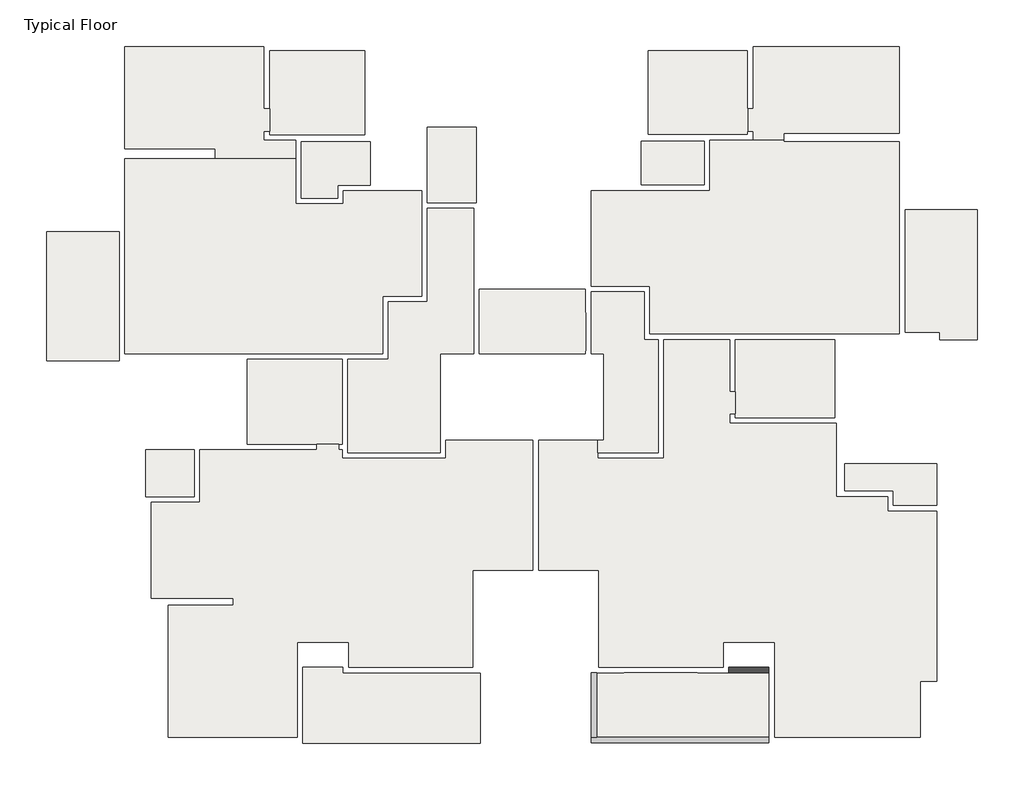
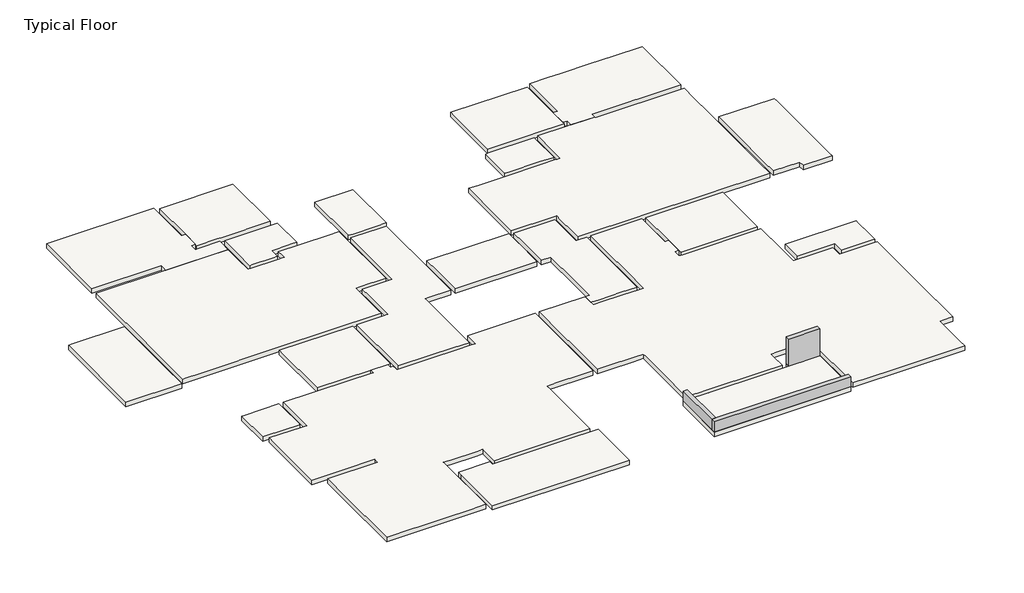
# One storey: 22 slabs, 3 beams.
"""IFC4 building model written with IfcOpenShell, lengths in millimetres."""

from ifc_helpers import new_model, si_unit, frame, origin, place, context, project, spatial, polyline, outline, extrude, faceted_brep, element, save

model = new_model("IFC4")

# Units and contexts
model_context = context("Model", 3, world=origin())
ifc_project = project(units=[si_unit("LENGTHUNIT", "METRE", prefix="MILLI")], contexts=[model_context])

# Site, building, storey
site = spatial("IfcSite", under=ifc_project)
building = spatial("IfcBuilding", under=site)
storey = spatial("IfcBuildingStorey", under=building, Name="Typical Floor", Elevation=3000.0)

# Beams
placement = place(None, origin())
element("IfcBeam", 1, ObjectType="Concrete Rectengular Beam : 20/133", at=placement, inside=storey, context=model_context, shape_type="Brep", body=[
    faceted_brep([(12927.905294, -11177.9835498, 4330.0), (12927.905294, -11177.9835498, 3000.0), (12927.905294, -11172.9835498, 3000.0), (12927.905294, -10977.9835498, 3000.0), (12927.905294, -10977.9835498, 4330.0), (11487.905294, -11177.9835498, 4330.0), (11487.905294, -10977.9835498, 4330.0), (11487.905294, -10977.9835498, 3000.0), (11487.905294, -11177.9835498, 3000.0)], [[[0, 1, 2, 3, 4]], [[5, 6, 7, 8]], [[4, 6, 5, 0]], [[3, 7, 6, 4]], [[1, 8, 7, 3, 2]], [[0, 5, 8, 1]]]),
])
element("IfcBeam", 2, ObjectType="Concrete Rectengular Beam : 20/50", at=placement, inside=storey, context=model_context, shape_type="Brep", body=[
    faceted_brep([(12927.905294, -13477.9835498, 3000.0), (12927.905294, -13477.9835498, 3500.0), (12927.905294, -13677.9835498, 3500.0), (12927.905294, -13677.9835498, 3000.0), (6765.405294, -13477.9835498, 3500.0), (6565.405294, -13477.9835498, 3500.0), (6565.405294, -13677.9835498, 3500.0), (6565.405294, -13677.9835498, 3000.0), (6565.405294, -13477.9835498, 3000.0), (6765.405294, -13477.9835498, 3000.0)], [[[0, 1, 2, 3]], [[2, 1, 4, 5, 6]], [[3, 2, 6, 7]], [[0, 3, 7, 8, 9]], [[1, 0, 9, 8, 5, 4]], [[6, 5, 8, 7]]]),
])
element("IfcBeam", 3, ObjectType="Concrete Rectengular Beam : 20/50", at=placement, inside=storey, context=model_context, shape_type="SweptSolid", body=[
    extrude(outline(polyline([(6565.405294, -11177.9835498), (6765.405294, -11177.9835498), (6765.405294, -13477.9835498), (6565.405294, -13477.9835498), (6565.405294, -11177.9835498)])), frame((0.0, 0.0, 3000.0), z_axis=(0.0, 0.0, 1.0), x_axis=(1.0, 0.0, 0.0)), (0.0, 0.0, 1.0), 500.0),
])

# Slabs
element("IfcSlab", 4, ObjectType="22", at=placement, inside=storey, context=model_context, shape_type="Brep", body=[
    faceted_brep([(2605.405294, -11177.9835498, 2780.0), (2605.405294, -13682.9835498, 2780.0), (-3754.594706, -13682.9835498, 2780.0), (-3754.594706, -11177.9835498, 2780.0), (-3754.594706, -10977.9835498, 2780.0), (-2314.594706, -10977.9835498, 2780.0), (-2314.594706, -11177.9835498, 2780.0), (-2114.594706, -11177.9835498, 2780.0), (-1184.594706, -11177.9835498, 2780.0), (1415.405294, -11177.9835498, 2780.0), (2605.405294, -13682.9835498, 3000.0), (2605.405294, -13482.9835498, 3000.0), (2605.405294, -11177.9835498, 3000.0), (2405.405294, -11177.9835498, 3000.0), (1415.405294, -11177.9835498, 3000.0), (-1184.594706, -11177.9835498, 3000.0), (-2114.594706, -11177.9835498, 3000.0), (-2314.594706, -11177.9835498, 3000.0), (-2314.594706, -10977.9835498, 3000.0), (-3754.594706, -10977.9835498, 3000.0), (-3754.594706, -11177.9835498, 3000.0), (-3754.594706, -13482.9835498, 3000.0), (-3754.594706, -13682.9835498, 3000.0)], [[[0, 1, 2, 3, 4, 5, 6, 7, 8, 9]], [[10, 11, 12, 13, 14, 15, 16, 17, 18, 19, 20, 21, 22]], [[1, 0, 12, 11, 10]], [[2, 1, 10, 22]], [[3, 2, 22, 21, 20]], [[4, 3, 20, 19]], [[5, 4, 19, 18]], [[6, 5, 18, 17]], [[6, 17, 16, 15, 14, 13, 12, 0, 9, 8, 7]]]),
])
element("IfcSlab", 5, ObjectType="22", at=placement, inside=storey, context=model_context, shape_type="Brep", body=[
    faceted_brep([(12927.905294, -13677.9835498, 2780.0), (6565.405294, -13677.9835498, 2780.0), (6565.405294, -11177.9835498, 2780.0), (7755.405294, -11177.9835498, 2780.0), (7755.405294, -11172.9835498, 2780.0), (10357.905294, -11172.9835498, 2780.0), (10357.905294, -11177.9835498, 2780.0), (11487.905294, -11177.9835498, 2780.0), (11487.905294, -10972.9835498, 2780.0), (12927.905294, -10972.9835498, 2780.0), (12927.905294, -11172.9835498, 2780.0), (6565.405294, -13677.9835498, 3000.0), (12927.905294, -13677.9835498, 3000.0), (12927.905294, -13477.9835498, 3000.0), (12927.905294, -11177.9835498, 3000.0), (12927.905294, -11172.9835498, 3000.0), (12927.905294, -10977.9835498, 3000.0), (12927.905294, -10972.9835498, 3000.0), (11487.905294, -10972.9835498, 3000.0), (11487.905294, -10977.9835498, 3000.0), (11487.905294, -11177.9835498, 3000.0), (10357.905294, -11177.9835498, 3000.0), (10357.905294, -11172.9835498, 3000.0), (7755.405294, -11172.9835498, 3000.0), (7755.405294, -11177.9835498, 3000.0), (6835.405294, -11177.9835498, 3000.0), (6765.405294, -11177.9835498, 3000.0), (6565.405294, -11177.9835498, 3000.0), (6565.405294, -13477.9835498, 3000.0)], [[[0, 1, 2, 3, 4, 5, 6, 7, 8, 9, 10]], [[11, 12, 13, 14, 15, 16, 17, 18, 19, 20, 21, 22, 23, 24, 25, 26, 27, 28]], [[1, 11, 28, 27, 2]], [[1, 0, 12, 11]], [[0, 10, 15, 14, 13, 12]], [[10, 9, 17, 16, 15]], [[17, 9, 8, 18]], [[4, 23, 22, 5]], [[2, 27, 26, 25, 24, 3]], [[3, 24, 23, 4]], [[6, 21, 20, 7]], [[21, 6, 5, 22]], [[7, 20, 19, 18, 8]]]),
])
element("IfcSlab", 6, ObjectType="22", at=placement, inside=storey, context=model_context, shape_type="Brep", body=[
    faceted_brep([(-4939.8370837, 11086.5624033, 2780.0), (-1534.8370837, 11086.5624033, 2780.0), (-1534.8370837, 8086.5624033, 2780.0), (-4939.8370837, 8086.5624033, 2780.0), (-4939.8370837, 8206.5624033, 2780.0), (-4939.8370837, 9006.5624033, 2780.0), (-1534.8370837, 11086.5624033, 3000.0), (-4939.8370837, 11086.5624033, 3000.0), (-4939.8370837, 9006.5624033, 3000.0), (-4939.8370837, 8206.5624033, 3000.0), (-4939.8370837, 8086.5624033, 3000.0), (-3999.8370837, 8086.5624033, 3000.0), (-3799.8370837, 8086.5624033, 3000.0), (-1534.8370837, 8086.5624033, 3000.0)], [[[0, 1, 2, 3, 4, 5]], [[6, 7, 8, 9, 10, 11, 12, 13]], [[1, 0, 7, 6]], [[1, 6, 13, 2]], [[7, 0, 5, 4, 3, 10, 9, 8]], [[10, 3, 2, 13, 12, 11]]]),
])
element("IfcSlab", 7, ObjectType="22", at=placement, inside=storey, context=model_context, shape_type="Brep", body=[
    faceted_brep([(-10119.6462524, 7575.1187953, 2780.0), (-10119.6462524, 11236.5624033, 2780.0), (-5139.8370837, 11236.5624033, 2780.0), (-5139.8370837, 9006.5624033, 2780.0), (-4939.8370837, 9006.5624033, 2780.0), (-4939.8370837, 8206.5624033, 2780.0), (-5139.8370837, 8206.5624033, 2780.0), (-5139.8370837, 7886.5624033, 2780.0), (-4939.8370837, 7886.5624033, 2780.0), (-3999.8370837, 7886.5624033, 2780.0), (-3999.8370837, 7215.1187953, 2780.0), (-6891.2699366, 7215.1187953, 2780.0), (-6891.2699366, 7575.1187953, 2780.0), (-10119.6462524, 11236.5624033, 3000.0), (-10119.6462524, 10130.5632806, 3000.0), (-10119.6462524, 8930.3987709, 3000.0), (-10119.6462524, 7575.1187953, 3000.0), (-6891.2699366, 7575.1187953, 3000.0), (-6891.2699366, 7215.1187953, 3000.0), (-3999.8370837, 7215.1187953, 3000.0), (-3999.8370837, 7726.5624033, 3000.0), (-3999.8370837, 7886.5624033, 3000.0), (-4939.8370837, 7886.5624033, 3000.0), (-5139.8370837, 7886.5624033, 3000.0), (-5139.8370837, 8206.5624033, 3000.0), (-4939.8370837, 8206.5624033, 3000.0), (-4939.8370837, 9006.5624033, 3000.0), (-5139.8370837, 9006.5624033, 3000.0), (-5139.8370837, 11236.5624033, 3000.0)], [[[0, 1, 2, 3, 4, 5, 6, 7, 8, 9, 10, 11, 12]], [[13, 14, 15, 16, 17, 18, 19, 20, 21, 22, 23, 24, 25, 26, 27, 28]], [[1, 0, 16, 15, 14, 13]], [[2, 1, 13, 28]], [[3, 2, 28, 27]], [[4, 3, 27, 26]], [[5, 4, 26, 25]], [[6, 5, 25, 24]], [[7, 6, 24, 23]], [[7, 23, 22, 21, 9, 8]], [[10, 9, 21, 20, 19]], [[11, 10, 19, 18]], [[12, 11, 18, 17]], [[0, 12, 17, 16]]]),
])
element("IfcSlab", 8, ObjectType="22", at=placement, inside=storey, context=model_context, shape_type="Brep", body=[
    faceted_brep([(508.320407, 6080.1520062, 2780.0), (508.320407, 2305.1520062, 2780.0), (-690.8131749, 2305.1520062, 2780.0), (-890.8131749, 2305.1520062, 2780.0), (-890.8131749, 1555.8429472, 2780.0), (-890.8131749, 556.7642019, 2780.0), (-890.8131749, 251.1884177, 2780.0), (-10119.6462524, 251.1884177, 2780.0), (-10119.6462524, 7215.1187953, 2780.0), (-6891.2699366, 7215.1187953, 2780.0), (-3999.8370837, 7215.1187953, 2780.0), (-3999.8370837, 6335.1520062, 2780.0), (-3999.8370837, 5815.1520062, 2780.0), (-3999.8370837, 5615.1520062, 2780.0), (-3696.679593, 5615.1520062, 2780.0), (-2696.679593, 5615.1520062, 2780.0), (-2301.679593, 5615.1520062, 2780.0), (-2301.679593, 5815.1520062, 2780.0), (-2301.679593, 6080.1520062, 2780.0), (-1171.679593, 6080.1520062, 2780.0), (28.320407, 6080.1520062, 2780.0), (508.320407, 2305.1520062, 3000.0), (508.320407, 6080.1520062, 3000.0), (28.320407, 6080.1520062, 3000.0), (-1171.679593, 6080.1520062, 3000.0), (-2301.679593, 6080.1520062, 3000.0), (-2301.679593, 5815.1520062, 3000.0), (-2301.679593, 5615.1520062, 3000.0), (-2696.679593, 5615.1520062, 3000.0), (-3696.679593, 5615.1520062, 3000.0), (-3999.8370837, 5615.1520062, 3000.0), (-3999.8370837, 5815.1520062, 3000.0), (-3999.8370837, 6335.1520062, 3000.0), (-3999.8370837, 7215.1187953, 3000.0), (-6891.2699366, 7215.1187953, 3000.0), (-10119.6462524, 7215.1187953, 3000.0), (-10119.6462524, 7055.0094311, 3000.0), (-10119.6462524, 5854.8449214, 3000.0), (-10119.6462524, 3780.4865094, 3000.0), (-10119.6462524, 1181.1884177, 3000.0), (-10119.6462524, 251.1884177, 3000.0), (-9999.6462524, 251.1884177, 3000.0), (-9290.9338154, 251.1884177, 3000.0), (-5740.9338154, 251.1884177, 3000.0), (-890.8131749, 251.1884177, 3000.0), (-890.8131749, 556.7642019, 3000.0), (-890.8131749, 1555.8429472, 3000.0), (-890.8131749, 2305.1520062, 3000.0), (-690.8131749, 2305.1520062, 3000.0)], [[[0, 1, 2, 3, 4, 5, 6, 7, 8, 9, 10, 11, 12, 13, 14, 15, 16, 17, 18, 19, 20]], [[21, 22, 23, 24, 25, 26, 27, 28, 29, 30, 31, 32, 33, 34, 35, 36, 37, 38, 39, 40, 41, 42, 43, 44, 45, 46, 47, 48]], [[30, 13, 12, 11, 10, 33, 32, 31]], [[13, 30, 29, 28, 27, 16, 15, 14]], [[16, 27, 26, 25, 18, 17]], [[18, 25, 24, 23, 22, 0, 20, 19]], [[1, 0, 22, 21]], [[1, 21, 48, 47, 3, 2]], [[3, 47, 46, 45, 44, 6, 5, 4]], [[7, 6, 44, 43, 42, 41, 40]], [[8, 7, 40, 39, 38, 37, 36, 35]], [[10, 9, 8, 35, 34, 33]]]),
])
element("IfcSlab", 9, ObjectType="22", at=placement, inside=storey, context=model_context, shape_type="Brep", body=[
    faceted_brep([(-12919.6462524, 4616.1884177, 2780.0), (-10319.6462524, 4616.1884177, 2780.0), (-10319.6462524, -12.6260152, 2780.0), (-12919.6462524, -12.6260152, 2780.0), (-12919.6462524, 4616.1884177, 3000.0), (-12919.6462524, 187.3739848, 3000.0), (-12919.6462524, -12.6260152, 3000.0), (-10319.6462524, -12.6260152, 3000.0), (-10319.6462524, 187.3739848, 3000.0), (-10319.6462524, 251.1884177, 3000.0), (-10319.6462524, 1181.1884177, 3000.0), (-10319.6462524, 3780.4865094, 3000.0), (-10319.6462524, 4416.1884177, 3000.0), (-10319.6462524, 4616.1884177, 3000.0), (-12719.6462524, 4616.1884177, 3000.0)], [[[0, 1, 2, 3]], [[4, 5, 6, 7, 8, 9, 10, 11, 12, 13, 14]], [[1, 0, 4, 14, 13]], [[2, 1, 13, 12, 11, 10, 9, 8, 7]], [[3, 2, 7, 6]], [[0, 3, 6, 5, 4]]]),
])
element("IfcSlab", 10, ObjectType="22", at=placement, inside=storey, context=model_context, shape_type="Brep", body=[
    faceted_brep([(-1339.8370837, 7836.5624033, 2780.0), (-1339.8370837, 6280.1520062, 2780.0), (-2301.679593, 6280.1520062, 2780.0), (-2501.679593, 6280.1520062, 2780.0), (-2501.679593, 5815.1520062, 2780.0), (-3799.8370837, 5815.1520062, 2780.0), (-3799.8370837, 7836.5624033, 2780.0), (-1339.8370837, 6280.1520062, 3000.0), (-1339.8370837, 7836.068874, 3000.0), (-1339.8370837, 7836.5624033, 3000.0), (-3799.8370837, 7836.5624033, 3000.0), (-3799.8370837, 7726.5624033, 3000.0), (-3799.8370837, 6335.1520062, 3000.0), (-3799.8370837, 5815.1520062, 3000.0), (-3696.679593, 5815.1520062, 3000.0), (-2696.679593, 5815.1520062, 3000.0), (-2501.679593, 5815.1520062, 3000.0), (-2501.679593, 6280.1520062, 3000.0), (-2301.679593, 6280.1520062, 3000.0), (-1489.8370837, 6280.1520062, 3000.0)], [[[0, 1, 2, 3, 4, 5, 6]], [[7, 8, 9, 10, 11, 12, 13, 14, 15, 16, 17, 18, 19]], [[1, 0, 9, 8, 7]], [[1, 7, 19, 18, 17, 3, 2]], [[4, 3, 17, 16]], [[5, 4, 16, 15, 14, 13]], [[6, 5, 13, 12, 11, 10]], [[0, 6, 10, 9]]]),
])
element("IfcSlab", 11, ObjectType="22", at=placement, inside=storey, context=model_context, shape_type="Brep", body=[
    faceted_brep([(8357.905294, 7842.0164502, 2780.0), (10617.905294, 7842.0164502, 2780.0), (10617.905294, 6284.3445962, 2780.0), (8357.905294, 6284.3445962, 2780.0), (8357.905294, 7842.0164502, 3000.0), (8357.905294, 6284.3445962, 3000.0), (8507.905294, 6284.3445962, 3000.0), (9959.9948169, 6284.3445962, 3000.0), (10569.9948169, 6284.3445962, 3000.0), (10617.905294, 6284.3445962, 3000.0), (10617.905294, 6354.3445962, 3000.0), (10617.905294, 7752.0164502, 3000.0), (10617.905294, 7842.0164502, 3000.0), (8507.905294, 7842.0164502, 3000.0)], [[[0, 1, 2, 3]], [[4, 5, 6, 7, 8, 9, 10, 11, 12, 13]], [[1, 0, 4, 13, 12]], [[2, 1, 12, 11, 10, 9]], [[3, 2, 9, 8, 7, 6, 5]], [[0, 3, 5, 4]]]),
])
element("IfcSlab", 12, ObjectType="22", at=placement, inside=storey, context=model_context, shape_type="Brep", body=[
    faceted_brep([(8607.905294, 8092.0164502, 2780.0), (8607.905294, 11082.0164502, 2780.0), (12157.905294, 11082.0164502, 2780.0), (12157.905294, 9012.0164502, 2780.0), (12162.905294, 9012.0164502, 2780.0), (12162.905294, 8212.0164502, 2780.0), (12157.905294, 8212.0164502, 2780.0), (12157.905294, 8092.0164502, 2780.0), (8607.905294, 11082.0164502, 3000.0), (8607.905294, 8092.0164502, 3000.0), (10617.905294, 8092.0164502, 3000.0), (10817.905294, 8092.0164502, 3000.0), (12157.905294, 8092.0164502, 3000.0), (12157.905294, 8212.0164502, 3000.0), (12162.905294, 8212.0164502, 3000.0), (12162.905294, 9012.0164502, 3000.0), (12157.905294, 9012.0164502, 3000.0), (12157.905294, 11082.0164502, 3000.0)], [[[0, 1, 2, 3, 4, 5, 6, 7]], [[8, 9, 10, 11, 12, 13, 14, 15, 16, 17]], [[4, 15, 14, 5]], [[9, 0, 7, 12, 11, 10]], [[1, 0, 9, 8]], [[1, 8, 17, 2]], [[16, 3, 2, 17]], [[3, 16, 15, 4]], [[6, 13, 12, 7]], [[13, 6, 5, 14]]]),
])
element("IfcSlab", 13, ObjectType="22", at=placement, inside=storey, context=model_context, shape_type="Brep", body=[
    faceted_brep([(12357.905294, 9012.0164502, 2780.0), (12357.905294, 11232.0164502, 2780.0), (17597.905294, 11232.0164502, 2780.0), (17597.905294, 8132.0164502, 2780.0), (13457.905294, 8132.0164502, 2780.0), (13457.905294, 7892.0164502, 2780.0), (12357.905294, 7892.0164502, 2780.0), (12357.905294, 8212.0164502, 2780.0), (12162.905294, 8212.0164502, 2780.0), (12162.905294, 9012.0164502, 2780.0), (12357.905294, 11232.0164502, 3000.0), (12357.905294, 9012.0164502, 3000.0), (12162.905294, 9012.0164502, 3000.0), (12162.905294, 8212.0164502, 3000.0), (12357.905294, 8212.0164502, 3000.0), (12357.905294, 7892.0164502, 3000.0), (13457.905294, 7892.0164502, 3000.0), (13457.905294, 8132.0164502, 3000.0), (17597.905294, 8132.0164502, 3000.0), (17597.905294, 11232.0164502, 3000.0), (16317.905294, 11232.0164502, 3000.0), (15097.905294, 11232.0164502, 3000.0), (13857.905294, 11232.0164502, 3000.0), (13257.905294, 11232.0164502, 3000.0)], [[[0, 1, 2, 3, 4, 5, 6, 7, 8, 9]], [[10, 11, 12, 13, 14, 15, 16, 17, 18, 19, 20, 21, 22, 23]], [[7, 14, 13, 8]], [[11, 0, 9, 12]], [[1, 0, 11, 10]], [[2, 1, 10, 23, 22, 21, 20, 19]], [[3, 2, 19, 18]], [[4, 3, 18, 17]], [[5, 4, 17, 16]], [[6, 5, 16, 15]], [[7, 6, 15, 14]], [[9, 8, 13, 12]]]),
])
element("IfcSlab", 14, ObjectType="22", at=placement, inside=storey, context=model_context, shape_type="Brep", body=[
    faceted_brep([(10817.905294, 7892.0164502, 2780.0), (12357.905294, 7892.0164502, 2780.0), (13457.905294, 7892.0164502, 2780.0), (13457.905294, 7832.0164502, 2780.0), (17597.905294, 7832.0164502, 2780.0), (17597.905294, 1022.0164502, 2780.0), (17597.905294, 952.0164502, 2780.0), (8663.320407, 952.0164502, 2780.0), (8663.320407, 1352.0164502, 2780.0), (8663.320407, 2355.1520062, 2780.0), (8663.320407, 2655.1520062, 2780.0), (8463.320407, 2655.1520062, 2780.0), (6563.320407, 2655.1520062, 2780.0), (6563.320407, 6084.3445962, 2780.0), (7043.320407, 6084.3445962, 2780.0), (8239.9948169, 6084.3445962, 2780.0), (9959.9948169, 6084.3445962, 2780.0), (10569.9948169, 6084.3445962, 2780.0), (10617.905294, 6084.3445962, 2780.0), (10817.905294, 6084.3445962, 2780.0), (10817.905294, 6354.3445962, 2780.0), (10817.905294, 7752.0164502, 2780.0), (13457.905294, 7892.0164502, 3000.0), (12357.905294, 7892.0164502, 3000.0), (12157.905294, 7892.0164502, 3000.0), (10817.905294, 7892.0164502, 3000.0), (10817.905294, 7752.0164502, 3000.0), (10817.905294, 6354.3445962, 3000.0), (10817.905294, 6084.3445962, 3000.0), (10617.905294, 6084.3445962, 3000.0), (10569.9948169, 6084.3445962, 3000.0), (9959.9948169, 6084.3445962, 3000.0), (8239.9948169, 6084.3445962, 3000.0), (7043.320407, 6084.3445962, 3000.0), (6563.320407, 6084.3445962, 3000.0), (6563.320407, 2655.1520062, 3000.0), (8463.320407, 2655.1520062, 3000.0), (8663.320407, 2655.1520062, 3000.0), (8663.320407, 2355.1520062, 3000.0), (8663.320407, 1352.0164502, 3000.0), (8663.320407, 952.0164502, 3000.0), (17597.905294, 952.0164502, 3000.0), (17597.905294, 1022.0164502, 3000.0), (17597.905294, 1732.0164502, 3000.0), (17597.905294, 4332.0164502, 3000.0), (17597.905294, 5872.0164502, 3000.0), (17597.905294, 7092.0164502, 3000.0), (17597.905294, 7832.0164502, 3000.0), (13457.905294, 7832.0164502, 3000.0)], [[[0, 1, 2, 3, 4, 5, 6, 7, 8, 9, 10, 11, 12, 13, 14, 15, 16, 17, 18, 19, 20, 21]], [[22, 23, 24, 25, 26, 27, 28, 29, 30, 31, 32, 33, 34, 35, 36, 37, 38, 39, 40, 41, 42, 43, 44, 45, 46, 47, 48]], [[28, 19, 18, 17, 16, 15, 14, 13, 34, 33, 32, 31, 30, 29]], [[19, 28, 27, 26, 25, 0, 21, 20]], [[2, 1, 0, 25, 24, 23, 22]], [[3, 2, 22, 48]], [[4, 3, 48, 47]], [[5, 4, 47, 46, 45, 44, 43, 42]], [[6, 5, 42, 41]], [[7, 6, 41, 40]], [[7, 40, 39, 38, 37, 10, 9, 8]], [[10, 37, 36, 35, 12, 11]], [[13, 12, 35, 34]]]),
])
element("IfcSlab", 15, ObjectType="22", at=placement, inside=storey, context=model_context, shape_type="Brep", body=[
    faceted_brep([(17797.905294, 5405.0203984, 2780.0), (20388.2392489, 5405.0203984, 2780.0), (20388.2392489, 1022.0164502, 2780.0), (20388.2392489, 752.0164502, 2780.0), (19037.905294, 752.0164502, 2780.0), (19037.905294, 1022.0164502, 2780.0), (17797.905294, 1022.0164502, 2780.0), (20388.2392489, 5405.0203984, 3000.0), (17797.905294, 5405.0203984, 3000.0), (17797.905294, 5205.0203984, 3000.0), (17797.905294, 4332.0164502, 3000.0), (17797.905294, 1732.0164502, 3000.0), (17797.905294, 1022.0164502, 3000.0), (19037.905294, 1022.0164502, 3000.0), (19037.905294, 752.0164502, 3000.0), (20188.2392489, 752.0164502, 3000.0), (20388.2392489, 752.0164502, 3000.0), (20388.2392489, 1022.0164502, 3000.0), (20388.2392489, 5205.0203984, 3000.0)], [[[0, 1, 2, 3, 4, 5, 6]], [[7, 8, 9, 10, 11, 12, 13, 14, 15, 16, 17, 18]], [[1, 0, 8, 7]], [[2, 1, 7, 18, 17]], [[6, 5, 13, 12]], [[0, 6, 12, 11, 10, 9, 8]], [[3, 2, 17, 16]], [[4, 3, 16, 15, 14]], [[5, 4, 14, 13]]]),
])
element("IfcSlab", 16, ObjectType="22", at=placement, inside=storey, context=model_context, shape_type="Brep", body=[
    faceted_brep([(2460.820407, 8355.1520062, 2780.0), (2460.820407, 5655.8758492, 2780.0), (708.320407, 5655.8758492, 2780.0), (708.320407, 8355.1520062, 2780.0), (2460.820407, 8355.1520062, 3000.0), (708.320407, 8355.1520062, 3000.0), (708.320407, 5655.8758492, 3000.0), (909.4061714, 5655.8758492, 3000.0), (2013.320407, 5655.8758492, 3000.0), (2460.820407, 5655.8758492, 3000.0)], [[[0, 1, 2, 3]], [[4, 5, 6, 7, 8, 9]], [[1, 0, 4, 9]], [[2, 1, 9, 8, 7, 6]], [[3, 2, 6, 5]], [[0, 3, 5, 4]]]),
])
element("IfcSlab", 17, ObjectType="22", at=placement, inside=storey, context=model_context, shape_type="Brep", body=[
    faceted_brep([(1160.820407, 252.3535615, 2780.0), (1160.820407, -3294.0144776, 2780.0), (-2136.5139865, -3294.0144776, 2780.0), (-2136.5139865, 51.1884177, 2780.0), (-890.8131749, 51.1884177, 2780.0), (-690.8131749, 51.1884177, 2780.0), (-690.8131749, 556.7642019, 2780.0), (-690.8131749, 1555.8429472, 2780.0), (-690.8131749, 2105.1520062, 2780.0), (708.320407, 2105.1520062, 2780.0), (708.320407, 2305.1520062, 2780.0), (708.320407, 5455.8758492, 2780.0), (2360.820407, 5455.8758492, 2780.0), (2360.820407, 1705.8758492, 2780.0), (2363.3932055, 1705.8758492, 2780.0), (2363.3932055, 352.3535615, 2780.0), (2360.820407, 352.3535615, 2780.0), (2360.820407, 252.3535615, 2780.0), (1360.820407, 252.3535615, 2780.0), (1160.820407, -3294.0144776, 3000.0), (1160.820407, 252.3535615, 3000.0), (1360.820407, 252.3535615, 3000.0), (2360.820407, 252.3535615, 3000.0), (2360.820407, 352.3535615, 3000.0), (2363.3932055, 352.3535615, 3000.0), (2363.3932055, 1705.8758492, 3000.0), (2360.820407, 1705.8758492, 3000.0), (2360.820407, 5455.8758492, 3000.0), (2013.320407, 5455.8758492, 3000.0), (909.4061714, 5455.8758492, 3000.0), (708.320407, 5455.8758492, 3000.0), (708.320407, 2305.1520062, 3000.0), (708.320407, 2105.1520062, 3000.0), (-690.8131749, 2105.1520062, 3000.0), (-690.8131749, 1555.8429472, 3000.0), (-690.8131749, 556.7642019, 3000.0), (-690.8131749, 51.1884177, 3000.0), (-890.8131749, 51.1884177, 3000.0), (-2136.5139865, 51.1884177, 3000.0), (-2136.5139865, -3294.0144776, 3000.0), (-591.3286388, -3294.0144776, 3000.0), (410.820407, -3294.0144776, 3000.0)], [[[0, 1, 2, 3, 4, 5, 6, 7, 8, 9, 10, 11, 12, 13, 14, 15, 16, 17, 18]], [[19, 20, 21, 22, 23, 24, 25, 26, 27, 28, 29, 30, 31, 32, 33, 34, 35, 36, 37, 38, 39, 40, 41]], [[14, 25, 24, 15]], [[20, 0, 18, 17, 22, 21]], [[1, 0, 20, 19]], [[2, 1, 19, 41, 40, 39]], [[3, 2, 39, 38]], [[3, 38, 37, 36, 5, 4]], [[5, 36, 35, 34, 33, 8, 7, 6]], [[9, 8, 33, 32]], [[9, 32, 31, 30, 11, 10]], [[11, 30, 29, 28, 27, 12]], [[26, 13, 12, 27]], [[13, 26, 25, 14]], [[16, 23, 22, 17]], [[23, 16, 15, 24]]]),
])
element("IfcSlab", 18, ObjectType="22", at=placement, inside=storey, context=model_context, shape_type="Brep", body=[
    faceted_brep([(2560.820407, 252.3535615, 2780.0), (2560.820407, 2545.8758492, 2780.0), (6363.320407, 2545.8758492, 2780.0), (6363.320407, 1705.1520062, 2780.0), (6368.320407, 1705.1520062, 2780.0), (6368.320407, 352.3535615, 2780.0), (6363.320407, 352.3535615, 2780.0), (6363.320407, 252.3535615, 2780.0), (2560.820407, 2545.8758492, 3000.0), (2560.820407, 1705.8758492, 3000.0), (2560.820407, 352.3535615, 3000.0), (2560.820407, 252.3535615, 3000.0), (6363.320407, 252.3535615, 3000.0), (6363.320407, 352.3535615, 3000.0), (6368.320407, 352.3535615, 3000.0), (6368.320407, 1705.1520062, 3000.0), (6363.320407, 1705.1520062, 3000.0), (6363.320407, 2545.8758492, 3000.0)], [[[0, 1, 2, 3, 4, 5, 6, 7]], [[8, 9, 10, 11, 12, 13, 14, 15, 16, 17]], [[4, 15, 14, 5]], [[11, 0, 7, 12]], [[1, 0, 11, 10, 9, 8]], [[1, 8, 17, 2]], [[16, 3, 2, 17]], [[3, 16, 15, 4]], [[6, 13, 12, 7]], [[13, 6, 5, 14]]]),
])
element("IfcSlab", 19, ObjectType="22", at=placement, inside=storey, context=model_context, shape_type="Brep", body=[
    faceted_brep([(8963.320407, 752.0164502, 2780.0), (8963.320407, -3297.9835498, 2780.0), (6810.820407, -3297.9835498, 2780.0), (6810.820407, -2847.6464385, 2780.0), (7010.820407, -2847.6464385, 2780.0), (7010.820407, -2447.6464385, 2780.0), (7010.820407, -1347.6464385, 2780.0), (7010.820407, 52.3535615, 2780.0), (7010.820407, 252.3535615, 2780.0), (6563.320407, 252.3535615, 2780.0), (6563.320407, 2455.1520062, 2780.0), (8463.320407, 2455.1520062, 2780.0), (8463.320407, 2355.1520062, 2780.0), (8463.320407, 1352.0164502, 2780.0), (8463.320407, 752.0164502, 2780.0), (8663.320407, 752.0164502, 2780.0), (8963.320407, -3297.9835498, 3000.0), (8963.320407, 752.0164502, 3000.0), (8663.320407, 752.0164502, 3000.0), (8463.320407, 752.0164502, 3000.0), (8463.320407, 1352.0164502, 3000.0), (8463.320407, 2355.1520062, 3000.0), (8463.320407, 2455.1520062, 3000.0), (6563.320407, 2455.1520062, 3000.0), (6563.320407, 1705.1520062, 3000.0), (6563.320407, 352.3535615, 3000.0), (6563.320407, 252.3535615, 3000.0), (7010.820407, 252.3535615, 3000.0), (7010.820407, 52.3535615, 3000.0), (7010.820407, -1347.6464385, 3000.0), (7010.820407, -2447.6464385, 3000.0), (7010.820407, -2847.6464385, 3000.0), (6810.820407, -2847.6464385, 3000.0), (6810.820407, -3297.9835498, 3000.0), (7210.820407, -3297.9835498, 3000.0), (8213.320407, -3297.9835498, 3000.0)], [[[0, 1, 2, 3, 4, 5, 6, 7, 8, 9, 10, 11, 12, 13, 14, 15]], [[16, 17, 18, 19, 20, 21, 22, 23, 24, 25, 26, 27, 28, 29, 30, 31, 32, 33, 34, 35]], [[19, 14, 13, 12, 11, 22, 21, 20]], [[14, 19, 18, 17, 0, 15]], [[1, 0, 17, 16]], [[2, 1, 16, 35, 34, 33]], [[3, 2, 33, 32]], [[4, 3, 32, 31]], [[4, 31, 30, 29, 28, 27, 8, 7, 6, 5]], [[9, 8, 27, 26]], [[10, 9, 26, 25, 24, 23]], [[11, 10, 23, 22]]]),
])
element("IfcSlab", 20, ObjectType="22", at=placement, inside=storey, context=model_context, shape_type="Brep", body=[
    faceted_brep([(-7634.594706, -3194.7427075, 2780.0), (-7634.594706, -4872.9835498, 2780.0), (-9365.9338154, -4872.9835498, 2780.0), (-9365.9338154, -3194.7427075, 2780.0), (-7634.594706, -3194.7427075, 3000.0), (-9214.7328942, -3194.7427075, 3000.0), (-9364.7328942, -3194.7427075, 3000.0), (-9365.9338154, -3194.7427075, 3000.0), (-9365.9338154, -4872.9835498, 3000.0), (-9364.7328942, -4872.9835498, 3000.0), (-9214.7328942, -4872.9835498, 3000.0), (-7634.594706, -4872.9835498, 3000.0), (-7634.594706, -4812.9835498, 3000.0), (-7634.594706, -3392.9835498, 3000.0)], [[[0, 1, 2, 3]], [[4, 5, 6, 7, 8, 9, 10, 11, 12, 13]], [[1, 0, 4, 13, 12, 11]], [[2, 1, 11, 10, 9, 8]], [[3, 2, 8, 7]], [[0, 3, 7, 6, 5, 4]]]),
])
element("IfcSlab", 21, ObjectType="22", at=placement, inside=storey, context=model_context, shape_type="Brep", body=[
    faceted_brep([(-5740.9338154, -2994.7427075, 2780.0), (-5740.9338154, 51.1884177, 2780.0), (-2336.5139865, 51.1884177, 2780.0), (-2336.5139865, -2994.0144776, 2780.0), (-2456.1345173, -2994.0144776, 2780.0), (-2456.1345173, -2994.7427075, 2780.0), (-3252.010806, -2994.7427075, 2780.0), (-5740.9338154, 51.1884177, 3000.0), (-5740.9338154, -18.8115823, 3000.0), (-5740.9338154, -2994.7427075, 3000.0), (-3252.010806, -2994.7427075, 3000.0), (-2456.1345173, -2994.7427075, 3000.0), (-2456.1345173, -2994.0144776, 3000.0), (-2336.5139865, -2994.0144776, 3000.0), (-2336.5139865, 51.1884177, 3000.0)], [[[0, 1, 2, 3, 4, 5, 6]], [[7, 8, 9, 10, 11, 12, 13, 14]], [[2, 14, 13, 3]], [[9, 0, 6, 5, 11, 10]], [[1, 0, 9, 8, 7]], [[2, 1, 7, 14]], [[12, 4, 3, 13]], [[4, 12, 11, 5]]]),
])
element("IfcSlab", 22, ObjectType="22", at=placement, inside=storey, context=model_context, shape_type="Brep", body=[
    faceted_brep([(15289.9526685, 752.0164502, 2780.0), (15289.9526685, -2047.9835498, 2780.0), (11717.905294, -2047.9835498, 2780.0), (11717.905294, -1907.9835498, 2780.0), (11717.905294, -1107.9835498, 2780.0), (11717.905294, 752.0164502, 2780.0), (15289.9526685, 752.0164502, 3000.0), (11717.905294, 752.0164502, 3000.0), (11717.905294, -1107.9835498, 3000.0), (11717.905294, -1907.9835498, 3000.0), (11717.905294, -2047.9835498, 3000.0), (15289.9526685, -2047.9835498, 3000.0)], [[[0, 1, 2, 3, 4, 5]], [[6, 7, 8, 9, 10, 11]], [[1, 0, 6, 11]], [[2, 1, 11, 10]], [[5, 4, 3, 2, 10, 9, 8, 7]], [[0, 5, 7, 6]]]),
])
element("IfcSlab", 23, ObjectType="22", at=placement, inside=storey, context=model_context, shape_type="Brep", body=[
    faceted_brep([(18937.905294, -3693.5538503, 2780.0), (18937.905294, -4662.9835498, 2780.0), (18937.905294, -5182.9835498, 2780.0), (17377.905294, -5182.9835498, 2780.0), (17377.905294, -4862.9835498, 2780.0), (17377.905294, -4662.9835498, 2780.0), (16897.905294, -4662.9835498, 2780.0), (16277.905294, -4662.9835498, 2780.0), (15639.9526685, -4662.9835498, 2780.0), (15639.9526685, -3693.5538503, 2780.0), (18937.905294, -4662.9835498, 3000.0), (18937.905294, -3843.5538503, 3000.0), (18937.905294, -3693.5538503, 3000.0), (15639.9526685, -3693.5538503, 3000.0), (15639.9526685, -3843.5538503, 3000.0), (15639.9526685, -4662.9835498, 3000.0), (16277.905294, -4662.9835498, 3000.0), (16897.905294, -4662.9835498, 3000.0), (17377.905294, -4662.9835498, 3000.0), (17377.905294, -4862.9835498, 3000.0), (17377.905294, -5182.9835498, 3000.0), (17457.905294, -5182.9835498, 3000.0), (18857.905294, -5182.9835498, 3000.0), (18937.905294, -5182.9835498, 3000.0)], [[[0, 1, 2, 3, 4, 5, 6, 7, 8, 9]], [[10, 11, 12, 13, 14, 15, 16, 17, 18, 19, 20, 21, 22, 23]], [[1, 0, 12, 11, 10]], [[2, 1, 10, 23]], [[3, 2, 23, 22, 21, 20]], [[3, 20, 19, 18, 5, 4]], [[5, 18, 17, 16, 15, 8, 7, 6]], [[9, 8, 15, 14, 13]], [[0, 9, 13, 12]]]),
])
element("IfcSlab", 24, ObjectType="22", at=placement, inside=storey, context=model_context, shape_type="Brep", body=[
    faceted_brep([(11517.905294, -1107.9835498, 2780.0), (11717.905294, -1107.9835498, 2780.0), (11717.905294, -1907.9835498, 2780.0), (11517.905294, -1907.9835498, 2780.0), (11517.905294, -2247.9835498, 2780.0), (11717.905294, -2247.9835498, 2780.0), (15339.9526685, -2247.9835498, 2780.0), (15339.9526685, -2447.9835498, 2780.0), (15339.9526685, -3647.9835498, 2780.0), (15339.9526685, -4662.9835498, 2780.0), (15339.9526685, -4862.9835498, 2780.0), (16277.905294, -4862.9835498, 2780.0), (16897.905294, -4862.9835498, 2780.0), (17177.905294, -4862.9835498, 2780.0), (17177.905294, -5182.9835498, 2780.0), (17177.905294, -5382.9835498, 2780.0), (17457.905294, -5382.9835498, 2780.0), (18857.905294, -5382.9835498, 2780.0), (18937.905294, -5382.9835498, 2780.0), (18937.905294, -11472.9835498, 2780.0), (18537.905294, -11472.9835498, 2780.0), (18337.905294, -11472.9835498, 2780.0), (18337.905294, -12447.9835498, 2780.0), (18337.905294, -13047.9835498, 2780.0), (18337.905294, -13477.9835498, 2780.0), (13127.905294, -13477.9835498, 2780.0), (13127.905294, -10277.9835498, 2780.0), (13127.905294, -10077.9835498, 2780.0), (12807.905294, -10077.9835498, 2780.0), (11607.905294, -10077.9835498, 2780.0), (11287.905294, -10077.9835498, 2780.0), (11287.905294, -10277.9835498, 2780.0), (11287.905294, -10977.9835498, 2780.0), (10357.905294, -10977.9835498, 2780.0), (7755.405294, -10977.9835498, 2780.0), (6835.405294, -10977.9835498, 2780.0), (6835.405294, -7702.9835498, 2780.0), (6835.405294, -7502.9835498, 2780.0), (6385.405294, -7502.9835498, 2780.0), (5185.405294, -7502.9835498, 2780.0), (4685.405294, -7502.9835498, 2780.0), (4685.405294, -2847.6464385, 2780.0), (6810.820407, -2847.6464385, 2780.0), (6810.820407, -3297.9835498, 2780.0), (6810.820407, -3497.9835498, 2780.0), (7210.820407, -3497.9835498, 2780.0), (8213.320407, -3497.9835498, 2780.0), (8963.320407, -3497.9835498, 2780.0), (9163.320407, -3497.9835498, 2780.0), (9163.320407, 752.0164502, 2780.0), (11517.905294, 752.0164502, 2780.0), (11717.905294, -1107.9835498, 3000.0), (11517.905294, -1107.9835498, 3000.0), (11517.905294, 752.0164502, 3000.0), (9163.320407, 752.0164502, 3000.0), (9163.320407, -3497.9835498, 3000.0), (8963.320407, -3497.9835498, 3000.0), (8213.320407, -3497.9835498, 3000.0), (7210.820407, -3497.9835498, 3000.0), (6810.820407, -3497.9835498, 3000.0), (6810.820407, -3297.9835498, 3000.0), (6810.820407, -2847.6464385, 3000.0), (4685.405294, -2847.6464385, 3000.0), (4685.405294, -7502.9835498, 3000.0), (5185.405294, -7502.9835498, 3000.0), (6385.405294, -7502.9835498, 3000.0), (6835.405294, -7502.9835498, 3000.0), (6835.405294, -7702.9835498, 3000.0), (6835.405294, -10977.9835498, 3000.0), (7755.405294, -10977.9835498, 3000.0), (10357.905294, -10977.9835498, 3000.0), (11287.905294, -10977.9835498, 3000.0), (11287.905294, -10277.9835498, 3000.0), (11287.905294, -10077.9835498, 3000.0), (11607.905294, -10077.9835498, 3000.0), (12807.905294, -10077.9835498, 3000.0), (13127.905294, -10077.9835498, 3000.0), (13127.905294, -10277.9835498, 3000.0), (13127.905294, -13477.9835498, 3000.0), (13857.905294, -13477.9835498, 3000.0), (15057.905294, -13477.9835498, 3000.0), (18337.905294, -13477.9835498, 3000.0), (18337.905294, -13047.9835498, 3000.0), (18337.905294, -12447.9835498, 3000.0), (18337.905294, -11472.9835498, 3000.0), (18537.905294, -11472.9835498, 3000.0), (18937.905294, -11472.9835498, 3000.0), (18937.905294, -8697.9835498, 3000.0), (18937.905294, -7497.9835498, 3000.0), (18937.905294, -5382.9835498, 3000.0), (18857.905294, -5382.9835498, 3000.0), (17457.905294, -5382.9835498, 3000.0), (17177.905294, -5382.9835498, 3000.0), (17177.905294, -5182.9835498, 3000.0), (17177.905294, -4862.9835498, 3000.0), (16897.905294, -4862.9835498, 3000.0), (16277.905294, -4862.9835498, 3000.0), (15339.9526685, -4862.9835498, 3000.0), (15339.9526685, -4662.9835498, 3000.0), (15339.9526685, -3647.9835498, 3000.0), (15339.9526685, -2447.9835498, 3000.0), (15339.9526685, -2247.9835498, 3000.0), (11717.905294, -2247.9835498, 3000.0), (11517.905294, -2247.9835498, 3000.0), (11517.905294, -1907.9835498, 3000.0), (11717.905294, -1907.9835498, 3000.0)], [[[0, 1, 2, 3, 4, 5, 6, 7, 8, 9, 10, 11, 12, 13, 14, 15, 16, 17, 18, 19, 20, 21, 22, 23, 24, 25, 26, 27, 28, 29, 30, 31, 32, 33, 34, 35, 36, 37, 38, 39, 40, 41, 42, 43, 44, 45, 46, 47, 48, 49, 50]], [[51, 52, 53, 54, 55, 56, 57, 58, 59, 60, 61, 62, 63, 64, 65, 66, 67, 68, 69, 70, 71, 72, 73, 74, 75, 76, 77, 78, 79, 80, 81, 82, 83, 84, 85, 86, 87, 88, 89, 90, 91, 92, 93, 94, 95, 96, 97, 98, 99, 100, 101, 102, 103, 104, 105]], [[1, 0, 52, 51]], [[2, 1, 51, 105]], [[3, 2, 105, 104]], [[4, 3, 104, 103]], [[4, 103, 102, 101, 6, 5]], [[6, 101, 100, 99, 98, 97, 10, 9, 8, 7]], [[10, 97, 96, 95, 94, 13, 12, 11]], [[13, 94, 93, 92, 15, 14]], [[15, 92, 91, 90, 89, 18, 17, 16]], [[19, 18, 89, 88, 87, 86]], [[19, 86, 85, 84, 21, 20]], [[21, 84, 83, 82, 81, 24, 23, 22]], [[25, 24, 81, 80, 79, 78]], [[25, 78, 77, 76, 27, 26]], [[27, 76, 75, 74, 73, 30, 29, 28]], [[30, 73, 72, 71, 32, 31]], [[32, 71, 70, 69, 68, 35, 34, 33]], [[35, 68, 67, 66, 37, 36]], [[37, 66, 65, 64, 63, 40, 39, 38]], [[41, 40, 63, 62]], [[42, 41, 62, 61]], [[42, 61, 60, 59, 44, 43]], [[44, 59, 58, 57, 56, 55, 48, 47, 46, 45]], [[49, 48, 55, 54]], [[50, 49, 54, 53]], [[0, 50, 53, 52]]]),
])
element("IfcSlab", 25, ObjectType="22", at=placement, inside=storey, context=model_context, shape_type="Brep", body=[
    faceted_brep([(-9164.594706, -8497.9835498, 2780.0), (-9164.594706, -5072.9835498, 2780.0), (-7634.594706, -5072.9835498, 2780.0), (-7434.594706, -5072.9835498, 2780.0), (-7434.594706, -4812.9835498, 2780.0), (-7434.594706, -3392.9835498, 2780.0), (-7434.594706, -3194.7427075, 2780.0), (-6090.9338154, -3194.7427075, 2780.0), (-5740.9338154, -3194.7427075, 2780.0), (-3252.010806, -3194.7427075, 2780.0), (-3252.010806, -2994.7427075, 2780.0), (-2456.1345173, -2994.7427075, 2780.0), (-2456.1345173, -3194.0144776, 2780.0), (-2336.5139865, -3194.0144776, 2780.0), (-2336.5139865, -3294.0144776, 2780.0), (-2336.5139865, -3494.0144776, 2780.0), (-591.3286388, -3494.0144776, 2780.0), (410.820407, -3494.0144776, 2780.0), (1160.820407, -3494.0144776, 2780.0), (1360.820407, -3494.0144776, 2780.0), (1360.820407, -2847.6464385, 2780.0), (4485.405294, -2847.6464385, 2780.0), (4485.405294, -7502.9835498, 2780.0), (3985.405294, -7502.9835498, 2780.0), (2785.405294, -7502.9835498, 2780.0), (2335.405294, -7502.9835498, 2780.0), (2335.405294, -7702.9835498, 2780.0), (2335.405294, -10977.9835498, 2780.0), (1415.405294, -10977.9835498, 2780.0), (-1184.594706, -10977.9835498, 2780.0), (-2114.594706, -10977.9835498, 2780.0), (-2114.594706, -10272.9835498, 2780.0), (-2114.594706, -10072.9835498, 2780.0), (-2434.594706, -10072.9835498, 2780.0), (-3634.594706, -10072.9835498, 2780.0), (-3954.594706, -10072.9835498, 2780.0), (-3954.594706, -10272.9835498, 2780.0), (-3954.594706, -13482.9835498, 2780.0), (-8564.594706, -13482.9835498, 2780.0), (-8564.594706, -10042.9835498, 2780.0), (-8564.594706, -9442.9835498, 2780.0), (-8564.594706, -8747.9835498, 2780.0), (-6234.594706, -8747.9835498, 2780.0), (-6234.594706, -8497.9835498, 2780.0), (-9164.594706, -5072.9835498, 3000.0), (-9164.594706, -7092.9835498, 3000.0), (-9164.594706, -8292.9835498, 3000.0), (-9164.594706, -8497.9835498, 3000.0), (-6234.594706, -8497.9835498, 3000.0), (-6234.594706, -8747.9835498, 3000.0), (-8564.594706, -8747.9835498, 3000.0), (-8564.594706, -9442.9835498, 3000.0), (-8564.594706, -10042.9835498, 3000.0), (-8564.594706, -13482.9835498, 3000.0), (-5884.594706, -13482.9835498, 3000.0), (-4664.594706, -13482.9835498, 3000.0), (-3954.594706, -13482.9835498, 3000.0), (-3954.594706, -10272.9835498, 3000.0), (-3954.594706, -10072.9835498, 3000.0), (-3634.594706, -10072.9835498, 3000.0), (-2434.594706, -10072.9835498, 3000.0), (-2114.594706, -10072.9835498, 3000.0), (-2114.594706, -10272.9835498, 3000.0), (-2114.594706, -10977.9835498, 3000.0), (-1184.594706, -10977.9835498, 3000.0), (1415.405294, -10977.9835498, 3000.0), (2335.405294, -10977.9835498, 3000.0), (2335.405294, -7702.9835498, 3000.0), (2335.405294, -7502.9835498, 3000.0), (2785.405294, -7502.9835498, 3000.0), (3985.405294, -7502.9835498, 3000.0), (4485.405294, -7502.9835498, 3000.0), (4485.405294, -2847.6464385, 3000.0), (1360.820407, -2847.6464385, 3000.0), (1360.820407, -3494.0144776, 3000.0), (1160.820407, -3494.0144776, 3000.0), (410.820407, -3494.0144776, 3000.0), (-591.3286388, -3494.0144776, 3000.0), (-2336.5139865, -3494.0144776, 3000.0), (-2336.5139865, -3294.0144776, 3000.0), (-2336.5139865, -3194.0144776, 3000.0), (-2456.1345173, -3194.0144776, 3000.0), (-2456.1345173, -2994.7427075, 3000.0), (-3252.010806, -2994.7427075, 3000.0), (-3252.010806, -3194.7427075, 3000.0), (-5740.9338154, -3194.7427075, 3000.0), (-6090.9338154, -3194.7427075, 3000.0), (-7434.594706, -3194.7427075, 3000.0), (-7434.594706, -3392.9835498, 3000.0), (-7434.594706, -4812.9835498, 3000.0), (-7434.594706, -5072.9835498, 3000.0), (-7634.594706, -5072.9835498, 3000.0)], [[[0, 1, 2, 3, 4, 5, 6, 7, 8, 9, 10, 11, 12, 13, 14, 15, 16, 17, 18, 19, 20, 21, 22, 23, 24, 25, 26, 27, 28, 29, 30, 31, 32, 33, 34, 35, 36, 37, 38, 39, 40, 41, 42, 43]], [[44, 45, 46, 47, 48, 49, 50, 51, 52, 53, 54, 55, 56, 57, 58, 59, 60, 61, 62, 63, 64, 65, 66, 67, 68, 69, 70, 71, 72, 73, 74, 75, 76, 77, 78, 79, 80, 81, 82, 83, 84, 85, 86, 87, 88, 89, 90, 91]], [[1, 0, 47, 46, 45, 44]], [[1, 44, 91, 90, 3, 2]], [[3, 90, 89, 88, 87, 6, 5, 4]], [[6, 87, 86, 85, 84, 9, 8, 7]], [[9, 84, 83, 10]], [[81, 12, 11, 82]], [[13, 12, 81, 80]], [[13, 80, 79, 78, 15, 14]], [[15, 78, 77, 76, 75, 74, 19, 18, 17, 16]], [[20, 19, 74, 73]], [[21, 20, 73, 72]], [[22, 21, 72, 71]], [[22, 71, 70, 69, 68, 25, 24, 23]], [[25, 68, 67, 66, 27, 26]], [[27, 66, 65, 64, 63, 30, 29, 28]], [[30, 63, 62, 61, 32, 31]], [[32, 61, 60, 59, 58, 35, 34, 33]], [[35, 58, 57, 56, 37, 36]], [[38, 37, 56, 55, 54, 53]], [[38, 53, 52, 51, 50, 41, 40, 39]], [[42, 41, 50, 49]], [[43, 42, 49, 48]], [[0, 43, 48, 47]], [[11, 10, 83, 82]]]),
])

save(model, "model.ifc")

# Revit data of these elements
# Type "Concrete Rectengular Beam : 20/133"
#   Length [instance default] = 152.4 cm
#   b = 20 cm
#   h = 133 cm
#   Structural Material [instance default] = Concrete
#   Assembly Code = ""
# Type "Concrete Rectengular Beam : 20/50"
#   Length [instance default] = 152.4 cm
#   b = 20 cm
#   h = 50 cm
#   Structural Material [instance default] = Concrete
#   Assembly Code = ""
# Type "22"
#   Function = 0
#   Layers, outside or top first: 22 cm "Concrete" (function 1)
# Element 1 (IfcBeam, "Concrete Rectengular Beam : 20/133")
#   Comments = ""
#   Mark = "B6"
#   SOFiSTiK_AMG_Comments = ""
#   SOFiSTiK_AMG_Scheduled = yes
#   SOFiSTiK_AMG_Adjusted = yes
#   Structural Material = Concrete
#   Phase Created = New Construction
#   Materials on its faces: "Concrete"
# Element 2 (IfcBeam, "Concrete Rectengular Beam : 20/50")
#   Comments = ""
#   Mark = "B32"
#   SOFiSTiK_AMG_Comments = ""
#   SOFiSTiK_AMG_Scheduled = yes
#   SOFiSTiK_AMG_Adjusted = yes
#   Structural Material = Concrete
#   Phase Created = New Construction
#   Materials on its faces: "Concrete"
# Element 3 (IfcBeam, "Concrete Rectengular Beam : 20/50")
#   Comments = ""
#   Mark = "B33"
#   SOFiSTiK_AMG_Comments = ""
#   SOFiSTiK_AMG_Scheduled = yes
#   SOFiSTiK_AMG_Adjusted = yes
#   Structural Material = Concrete
#   Phase Created = New Construction
#   Materials on its faces: "Concrete"
# Element 4 (IfcSlab, "22")
#   Mark = "S1"
#   SOFiSTiK_AMG_Comments = ""
#   built-in parameter 1001955 = 1.5708 (stored number, unit not read)
#   Height Offset From Level = 0 cm
#   built-in parameter 1001954 = 1
#   SOFiSTiK_AMG_Scheduled = yes
#   SOFiSTiK_AMG_Adjusted = yes
#   Phase Created = New Construction
#   Materials on its faces: "Concrete"
# Element 5 (IfcSlab, "22")
#   Mark = "S2"
#   SOFiSTiK_AMG_Comments = ""
#   built-in parameter 1001955 = 1.5708 (stored number, unit not read)
#   Height Offset From Level = 0 cm
#   built-in parameter 1001954 = 1
#   SOFiSTiK_AMG_Scheduled = yes
#   SOFiSTiK_AMG_Adjusted = yes
#   Phase Created = New Construction
#   Materials on its faces: "Concrete"
# Element 6 (IfcSlab, "22")
#   Mark = "S3"
#   SOFiSTiK_AMG_Comments = ""
#   built-in parameter 1001955 = 3.14159 (stored number, unit not read)
#   Height Offset From Level = 0 cm
#   built-in parameter 1001954 = 1
#   SOFiSTiK_AMG_Scheduled = yes
#   SOFiSTiK_AMG_Adjusted = yes
#   Phase Created = New Construction
#   Materials on its faces: "Concrete"
# Element 7 (IfcSlab, "22")
#   Mark = "S4"
#   SOFiSTiK_AMG_Comments = ""
#   built-in parameter 1001955 = -1.5708 (stored number, unit not read)
#   Height Offset From Level = 0 cm
#   built-in parameter 1001954 = 1
#   SOFiSTiK_AMG_Scheduled = yes
#   SOFiSTiK_AMG_Adjusted = yes
#   Phase Created = New Construction
#   Materials on its faces: "Concrete"
# Element 8 (IfcSlab, "22")
#   Mark = "S5"
#   SOFiSTiK_AMG_Comments = ""
#   Height Offset From Level = 0 cm
#   built-in parameter 1001954 = 1
#   SOFiSTiK_AMG_Scheduled = yes
#   SOFiSTiK_AMG_Adjusted = yes
#   Phase Created = New Construction
#   Materials on its faces: "Concrete"
# Element 9 (IfcSlab, "22")
#   Mark = "S6"
#   SOFiSTiK_AMG_Comments = ""
#   built-in parameter 1001955 = 3.14159 (stored number, unit not read)
#   Height Offset From Level = 0 cm
#   built-in parameter 1001954 = 1
#   SOFiSTiK_AMG_Scheduled = yes
#   SOFiSTiK_AMG_Adjusted = yes
#   Phase Created = New Construction
#   Materials on its faces: "Concrete"
# Element 10 (IfcSlab, "22")
#   Mark = "S7"
#   SOFiSTiK_AMG_Comments = ""
#   Height Offset From Level = 0 cm
#   built-in parameter 1001954 = 1
#   SOFiSTiK_AMG_Scheduled = yes
#   SOFiSTiK_AMG_Adjusted = yes
#   Phase Created = New Construction
#   Materials on its faces: "Concrete"
# Element 11 (IfcSlab, "22")
#   Mark = "S8"
#   SOFiSTiK_AMG_Comments = ""
#   built-in parameter 1001955 = 1.5708 (stored number, unit not read)
#   Height Offset From Level = 0 cm
#   built-in parameter 1001954 = 1
#   SOFiSTiK_AMG_Scheduled = yes
#   SOFiSTiK_AMG_Adjusted = yes
#   Phase Created = New Construction
#   Materials on its faces: "Concrete"
# Element 12 (IfcSlab, "22")
#   Mark = "S9"
#   SOFiSTiK_AMG_Comments = ""
#   Height Offset From Level = 0 cm
#   built-in parameter 1001954 = 1
#   SOFiSTiK_AMG_Scheduled = yes
#   SOFiSTiK_AMG_Adjusted = yes
#   Phase Created = New Construction
#   Materials on its faces: "Concrete"
# Element 13 (IfcSlab, "22")
#   Mark = "S10"
#   SOFiSTiK_AMG_Comments = ""
#   Height Offset From Level = 0 cm
#   built-in parameter 1001954 = 1
#   SOFiSTiK_AMG_Scheduled = yes
#   SOFiSTiK_AMG_Adjusted = yes
#   Phase Created = New Construction
#   Materials on its faces: "Concrete"
# Element 14 (IfcSlab, "22")
#   Mark = "S11"
#   SOFiSTiK_AMG_Comments = ""
#   built-in parameter 1001955 = 1.5708 (stored number, unit not read)
#   Height Offset From Level = 0 cm
#   built-in parameter 1001954 = 1
#   SOFiSTiK_AMG_Scheduled = yes
#   SOFiSTiK_AMG_Adjusted = yes
#   Phase Created = New Construction
#   Materials on its faces: "Concrete"
# Element 15 (IfcSlab, "22")
#   Mark = "S12"
#   SOFiSTiK_AMG_Comments = ""
#   built-in parameter 1001955 = 3.14159 (stored number, unit not read)
#   Height Offset From Level = 0 cm
#   built-in parameter 1001954 = 1
#   SOFiSTiK_AMG_Scheduled = yes
#   SOFiSTiK_AMG_Adjusted = yes
#   Phase Created = New Construction
#   Materials on its faces: "Concrete"
# Element 16 (IfcSlab, "22")
#   Mark = "S13"
#   SOFiSTiK_AMG_Comments = ""
#   Height Offset From Level = 0 cm
#   built-in parameter 1001954 = 1
#   SOFiSTiK_AMG_Scheduled = yes
#   SOFiSTiK_AMG_Adjusted = yes
#   Phase Created = New Construction
#   Materials on its faces: "Concrete"
# Element 17 (IfcSlab, "22")
#   Mark = "S14"
#   SOFiSTiK_AMG_Comments = ""
#   Height Offset From Level = 0 cm
#   built-in parameter 1001954 = 1
#   SOFiSTiK_AMG_Scheduled = yes
#   SOFiSTiK_AMG_Adjusted = yes
#   Phase Created = New Construction
#   Materials on its faces: "Concrete"
# Element 18 (IfcSlab, "22")
#   Mark = "S15"
#   SOFiSTiK_AMG_Comments = ""
#   Height Offset From Level = 0 cm
#   built-in parameter 1001954 = 1
#   SOFiSTiK_AMG_Scheduled = yes
#   SOFiSTiK_AMG_Adjusted = yes
#   Phase Created = New Construction
#   Materials on its faces: "Concrete"
# Element 19 (IfcSlab, "22")
#   Mark = "S16"
#   SOFiSTiK_AMG_Comments = ""
#   Height Offset From Level = 0 cm
#   built-in parameter 1001954 = 1
#   SOFiSTiK_AMG_Scheduled = yes
#   SOFiSTiK_AMG_Adjusted = yes
#   Phase Created = New Construction
#   Materials on its faces: "Concrete"
# Element 20 (IfcSlab, "22")
#   Mark = "S17"
#   SOFiSTiK_AMG_Comments = ""
#   Height Offset From Level = 0 cm
#   built-in parameter 1001954 = 1
#   SOFiSTiK_AMG_Scheduled = yes
#   SOFiSTiK_AMG_Adjusted = yes
#   Phase Created = New Construction
#   Materials on its faces: "Concrete"
# Element 21 (IfcSlab, "22")
#   Mark = "S18"
#   SOFiSTiK_AMG_Comments = ""
#   Height Offset From Level = 0 cm
#   built-in parameter 1001954 = 1
#   SOFiSTiK_AMG_Scheduled = yes
#   SOFiSTiK_AMG_Adjusted = yes
#   Phase Created = New Construction
#   Materials on its faces: "Concrete"
# Element 22 (IfcSlab, "22")
#   Mark = "S19"
#   SOFiSTiK_AMG_Comments = ""
#   Height Offset From Level = 0 cm
#   built-in parameter 1001954 = 1
#   SOFiSTiK_AMG_Scheduled = yes
#   SOFiSTiK_AMG_Adjusted = yes
#   Phase Created = New Construction
#   Materials on its faces: "Concrete"
# Element 23 (IfcSlab, "22")
#   Mark = "S20"
#   SOFiSTiK_AMG_Comments = ""
#   Height Offset From Level = 0 cm
#   built-in parameter 1001954 = 1
#   SOFiSTiK_AMG_Scheduled = yes
#   SOFiSTiK_AMG_Adjusted = yes
#   Phase Created = New Construction
#   Materials on its faces: "Concrete"
# Element 24 (IfcSlab, "22")
#   Mark = "S21"
#   SOFiSTiK_AMG_Comments = ""
#   built-in parameter 1001955 = -1.5708 (stored number, unit not read)
#   Height Offset From Level = 0 cm
#   built-in parameter 1001954 = 1
#   SOFiSTiK_AMG_Scheduled = yes
#   SOFiSTiK_AMG_Adjusted = yes
#   Phase Created = New Construction
#   Materials on its faces: "Concrete"
# Element 25 (IfcSlab, "22")
#   Mark = "S22"
#   SOFiSTiK_AMG_Comments = ""
#   built-in parameter 1001955 = -1.5708 (stored number, unit not read)
#   Height Offset From Level = 0 cm
#   built-in parameter 1001954 = 1
#   SOFiSTiK_AMG_Scheduled = yes
#   SOFiSTiK_AMG_Adjusted = yes
#   Phase Created = New Construction
#   Materials on its faces: "Concrete"
# Materials
#   "Concrete": class "Concrete", colour RGB 192 192 192, transparency 0, Keynote = "01000", Description = "Cast-in-place concrete", Cost = 0
